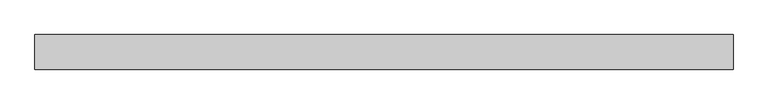
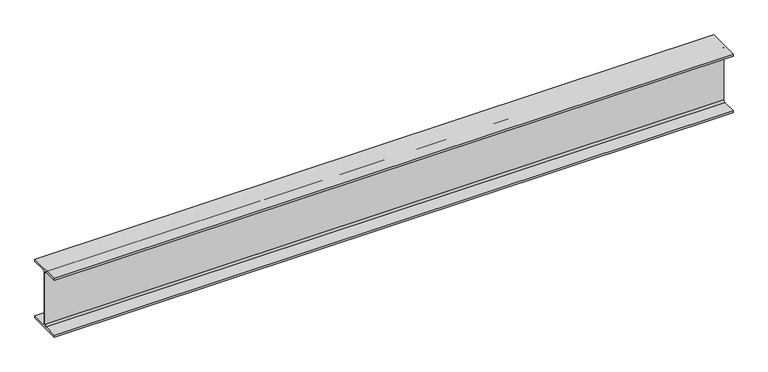
"""IFC4 building model written with IfcOpenShell, lengths in millimetres: beam geometry, Old_Steel Beam_H-KSD3502 : H_SB_ASB_H-200×200x8x12."""

import ifcopenshell
import ifcopenshell.guid

model = None  # the IFC model being written
_history = None  # IfcOwnerHistory: only IFC2X3 demands one
_inside = {}  # id of a spatial element -> (the spatial element, [elements in it])
_under = {}  # id of a project, library or spatial element -> (it, [spatial elements below it])
_declared = {}  # id of a project -> (the project, [libraries it declares])
_typed = {}  # id of a type object -> (the type object, [elements of that type])
_made_of = {}  # id of a material, layer set ... -> (it, [elements and type objects made of it])


def new_model(schema):
    """Start an empty IFC model of exactly this schema.

    Asked for "IFC4X3", IfcOpenShell would pick the latest addendum, in which some entities
    have other attributes; the version numbers below select the first issue.
    IFC2X3 requires an IfcOwnerHistory on every rooted entity: one is made here for all.
    """
    global model, _history
    if schema == "IFC4X3":
        model = ifcopenshell.file(schema_version=(4, 3, 0, 0))
    else:
        model = ifcopenshell.file(schema=schema)
    _inside.clear()
    _under.clear()
    _declared.clear()
    _typed.clear()
    _made_of.clear()
    _history = None
    if model.schema == "IFC2X3":
        org = make("IfcOrganization", Name="unknown")
        user = make(
            "IfcPersonAndOrganization",
            ThePerson=make("IfcPerson", FamilyName="unknown"),
            TheOrganization=org,
        )
        app = make(
            "IfcApplication",
            ApplicationDeveloper=org,
            Version="unknown",
            ApplicationFullName="unknown",
            ApplicationIdentifier="unknown",
        )
        _history = make(
            "IfcOwnerHistory",
            OwningUser=user,
            OwningApplication=app,
            ChangeAction="ADDED",
            CreationDate=0,
        )
    return model


def make(cls, **values):
    """One entity of the class cls with the attributes given. An attribute that is None is left unset."""
    return model.create_entity(
        cls, **{name: value for name, value in values.items() if value is not None}
    )


def rooted(cls, **values):
    """An entity with a GlobalId (a new one), such as an element, a storey or a relation."""
    return make(cls, GlobalId=ifcopenshell.guid.new(), OwnerHistory=_history, **values)


def si_unit(unit_type, name, prefix=None):
    """IfcSIUnit, for example si_unit("LENGTHUNIT", "METRE", prefix="MILLI")."""
    return make("IfcSIUnit", UnitType=unit_type, Prefix=prefix, Name=name)


def assignment(units):
    """IfcUnitAssignment: the units of a project."""
    return None if units is None else make("IfcUnitAssignment", Units=units)


def point(xyz):
    """IfcCartesianPoint."""
    return None if xyz is None else make("IfcCartesianPoint", Coordinates=xyz)


def direction(xyz):
    """IfcDirection."""
    return None if xyz is None else make("IfcDirection", DirectionRatios=xyz)


def frame(location, z_axis=None, x_axis=None):
    """IfcAxis2Placement3D, a coordinate frame: its origin and axes. An axis left out is left unset."""
    return make(
        "IfcAxis2Placement3D",
        Location=point(location),
        Axis=direction(z_axis),
        RefDirection=direction(x_axis),
    )


def frame_2d(location, x_axis=None):
    """IfcAxis2Placement2D, a coordinate frame in the plane: its origin and x axis."""
    return make(
        "IfcAxis2Placement2D", Location=point(location), RefDirection=direction(x_axis)
    )


def origin():
    """The frame at (0, 0, 0) with its axes left unset."""
    return frame((0.0, 0.0, 0.0))


def place(relative_to, where):
    """IfcLocalPlacement: puts the frame where relative to a parent placement (None: the world)."""
    return make(
        "IfcLocalPlacement", PlacementRelTo=relative_to, RelativePlacement=where
    )


def context(
    kind, dimensions, precision=None, world=None, true_north=None, identifier=None
):
    """IfcGeometricRepresentationContext, for example the 3D "Model" context."""
    return make(
        "IfcGeometricRepresentationContext",
        ContextIdentifier=identifier,
        ContextType=kind,
        CoordinateSpaceDimension=dimensions,
        Precision=precision,
        WorldCoordinateSystem=world,
        TrueNorth=true_north,
    )


def project(units=None, contexts=None):
    """IfcProject with its units and contexts."""
    return rooted(
        "IfcProject",
        Name="project",
        RepresentationContexts=contexts,
        UnitsInContext=assignment(units),
    )


def spatial(cls, under=None, at=None, **own):
    """A site, building, storey or space (cls), placed at a placement, below another one or the project."""
    s = rooted(cls, ObjectPlacement=at, **own)
    if under is not None:
        _under.setdefault(under.id(), (under, []))[1].append(s)
    return s


def polyline(points):
    """IfcPolyline through the points."""
    return make("IfcPolyline", Points=[point(p) for p in points])


def circle_curve(where, radius):
    """IfcCircle in the frame where."""
    return make("IfcCircle", Position=where, Radius=radius)


def trimmed(basis, trim1, trim2, sense, master):
    """IfcTrimmedCurve: the piece of a basis curve between two trims."""
    return make(
        "IfcTrimmedCurve",
        BasisCurve=basis,
        Trim1=trim1,
        Trim2=trim2,
        SenseAgreement=sense,
        MasterRepresentation=master,
    )


def segment(curve, same_sense, transition):
    """IfcCompositeCurveSegment."""
    return make(
        "IfcCompositeCurveSegment",
        Transition=transition,
        SameSense=same_sense,
        ParentCurve=curve,
    )


def composite_curve(segments, self_intersect=None):
    """IfcCompositeCurve: segments joined end to end."""
    return make("IfcCompositeCurve", Segments=segments, SelfIntersect=self_intersect)


def outline(outer, holes=None, kind="AREA"):
    """IfcArbitraryClosedProfileDef: a profile drawn as a closed curve; with holes, ...WithVoids."""
    if holes is None:
        return make("IfcArbitraryClosedProfileDef", ProfileType=kind, OuterCurve=outer)
    return make(
        "IfcArbitraryProfileDefWithVoids",
        ProfileType=kind,
        OuterCurve=outer,
        InnerCurves=holes,
    )


def extrude(swept, where, along, depth):
    """IfcExtrudedAreaSolid: the profile swept, set in the frame where, extruded along a direction by depth."""
    return make(
        "IfcExtrudedAreaSolid",
        SweptArea=swept,
        Position=where,
        ExtrudedDirection=direction(along),
        Depth=depth,
    )


def shape(context_of_items, identifier, shape_type, items):
    """IfcShapeRepresentation: the items that make up one representation, for example the "Body"."""
    return make(
        "IfcShapeRepresentation",
        ContextOfItems=context_of_items,
        RepresentationIdentifier=identifier,
        RepresentationType=shape_type,
        Items=items,
    )


def source(mapping_origin, context_of_items, identifier, shape_type, items):
    """IfcRepresentationMap: a shape defined once, which mapped items show again and again."""
    return make(
        "IfcRepresentationMap",
        MappingOrigin=mapping_origin,
        MappedRepresentation=shape(context_of_items, identifier, shape_type, items),
    )


def transform(
    local_origin,
    x_axis=None,
    y_axis=None,
    z_axis=None,
    scale=None,
    scale2=None,
    scale3=None,
    uniform=True,
):
    """IfcCartesianTransformationOperator3D, or its non-uniform kind. x_axis, y_axis, z_axis: its Axis1, 2, 3."""
    if uniform:
        return make(
            "IfcCartesianTransformationOperator3D",
            Axis1=direction(x_axis),
            Axis2=direction(y_axis),
            LocalOrigin=point(local_origin),
            Scale=scale,
            Axis3=direction(z_axis),
        )
    return make(
        "IfcCartesianTransformationOperator3DnonUniform",
        Axis1=direction(x_axis),
        Axis2=direction(y_axis),
        LocalOrigin=point(local_origin),
        Scale=scale,
        Axis3=direction(z_axis),
        Scale2=scale2,
        Scale3=scale3,
    )


def mapped(mapping_source, mapping_target):
    """IfcMappedItem: shows the shape of a source again, moved by a transform."""
    return make(
        "IfcMappedItem", MappingSource=mapping_source, MappingTarget=mapping_target
    )


def made_of(thing, what):
    """Note that an element or type object is made of a material, layer set ...; save() writes the relation."""
    if what is not None:
        _made_of.setdefault(what.id(), (what, []))[1].append(thing)
    return thing


def element(
    cls,
    number,
    at=None,
    inside=None,
    cuts=None,
    type_object=None,
    material=None,
    context=None,
    identifier="Body",
    shape_type=None,
    held_by="IfcProductDefinitionShape",
    body=None,
    shapes=None,
    **own,
):
    """One element of the class cls, such as IfcWall. Its Tag is "e" and its number.

    at: its placement. inside: the storey or other place that contains it. cuts: it is an
    opening in that element (IfcRelVoidsElement). A single representation is given by context,
    identifier, shape_type and body (its items); several are given by shapes. held_by: the class
    of the entity that holds the representations. save() writes the other relations.
    """
    e = rooted(cls, Tag="e%d" % number, ObjectPlacement=at, **own)
    if body is not None:
        shapes = [shape(context, identifier, shape_type, body)]
    if shapes is not None:
        e.Representation = make(held_by, Representations=shapes)
    if inside is not None:
        _inside.setdefault(inside.id(), (inside, []))[1].append(e)
    if cuts is not None:
        rooted(
            "IfcRelVoidsElement", RelatingBuildingElement=cuts, RelatedOpeningElement=e
        )
    if type_object is not None:
        _typed.setdefault(type_object.id(), (type_object, []))[1].append(e)
    return made_of(e, material)


def aggregate(whole, parts):
    """IfcRelAggregates: a whole, such as a stair, and the parts it consists of."""
    return rooted("IfcRelAggregates", RelatingObject=whole, RelatedObjects=parts)


def save(model, path):
    """Write the relations noted so far, then the file.

    IfcRelAggregates (storeys below a building ...), IfcRelContainedInSpatialStructure (elements
    in a storey), IfcRelDefinesByType, IfcRelAssociatesMaterial and IfcRelDeclares: one each for
    every whole, place, type object, material and project.
    """
    for whole, parts in _under.values():
        aggregate(whole, parts)
    for where, things in _inside.values():
        rooted(
            "IfcRelContainedInSpatialStructure",
            RelatedElements=things,
            RelatingStructure=where,
        )
    for kind, things in _typed.values():
        rooted("IfcRelDefinesByType", RelatedObjects=things, RelatingType=kind)
    for what, things in _made_of.values():
        rooted("IfcRelAssociatesMaterial", RelatedObjects=things, RelatingMaterial=what)
    for by, libraries in _declared.values():
        rooted("IfcRelDeclares", RelatingContext=by, RelatedDefinitions=libraries)
    model.write(path)


def beam_fe0ad751(model_context):
    return source(origin(), model_context, "Body", "SweptSolid", [
        extrude(outline(composite_curve([segment(polyline([(82.5, -141.5), (82.5, -151.7), (-82.5, -151.7), (-82.5, -141.5), (-11.9, -141.5)]), True, "CONTINUOUS"), segment(trimmed(circle_curve(frame_2d((-11.9, -132.6)), 8.9), [point((-11.9, -141.5))], [point((-3.0, -132.6))], True, "CARTESIAN"), True, "CONTINUOUS"), segment(polyline([(-3.0, -132.6), (-3.0, 132.6)]), True, "CONTINUOUS"), segment(trimmed(circle_curve(frame_2d((-11.9, 132.6)), 8.9), [point((-3.0, 132.6))], [point((-11.9, 141.5))], True, "CARTESIAN"), True, "CONTINUOUS"), segment(polyline([(-11.9, 141.5), (-82.5, 141.5), (-82.5, 151.7), (82.5, 151.7), (82.5, 141.5), (11.9, 141.5)]), True, "CONTINUOUS"), segment(trimmed(circle_curve(frame_2d((11.9, 132.6)), 8.9), [point((11.9, 141.5))], [point((3.0, 132.6))], True, "CARTESIAN"), True, "CONTINUOUS"), segment(polyline([(3.0, 132.6), (3.0, -132.6)]), True, "CONTINUOUS"), segment(trimmed(circle_curve(frame_2d((11.9, -132.6)), 8.9), [point((3.0, -132.6))], [point((11.9, -141.5))], True, "CARTESIAN"), True, "CONTINUOUS"), segment(polyline([(11.9, -141.5), (82.5, -141.5)]), True, "CONTINUOUS")], self_intersect=False)), frame((-1716.7775834, 0.0, 0.0), z_axis=(1.0, 0.0, 0.0), x_axis=(0.0, 1.0, 0.0)), (0.0, 0.0, 1.0), 3324.8852978),
    ])


if __name__ == "__main__":
    model = new_model("IFC4")
    model_context = context("Model", 3, world=origin())
    ifc_project = project(units=[si_unit("LENGTHUNIT", "METRE", prefix="MILLI")], contexts=[model_context])
    site = spatial("IfcSite", under=ifc_project)
    building = spatial("IfcBuilding", under=site)
    placement = place(None, origin())
    beam_shape = beam_fe0ad751(model_context)
    element("IfcBeam", 1, ObjectType="Old_Steel Beam_H-KSD3502 : H_SB_ASB_H-200×200x8x12", at=placement, inside=building, context=model_context, shape_type="MappedRepresentation", body=[
        mapped(beam_shape, transform((0.0, 0.0, 0.0), x_axis=(1.0, 0.0, 0.0), y_axis=(0.0, 1.0, 0.0), z_axis=(0.0, 0.0, 1.0))),
    ])
    save(model, "model.ifc")

# Revit data of these elements
# Type "Old_Steel Beam_H-KSD3502 : H_SB_ASB_H-200×200x8x12"
#   Width = 20.0 cm
#   Web Thickness = 0.8 cm
#   Web Fillet = 1.3 cm
#   Warping Constant = 141376.0 cm⁶
#   Torsional Moment of Inertia = 26.2485 cm⁴
#   Torsional Modulus = 1.0 cm³
#   Section Area = 63.53 cm²
#   Plastic Modulus weak axis = 244.0 cm³
#   Plastic Modulus strong axis = 525.0 cm³
#   Perimeter = 1.16 m²/m
#   Nominal Weight = 49.90 kgf/m
#   Moment of Inertia weak axis = 1600.00 cm⁴
#   Moment of Inertia strong axis = 4720.00 cm⁴
#   Height = 20.0 cm
#   Flange Thickness = 1.2 cm
#   Elastic Modulus weak axis = 160.0 cm³
#   Elastic Modulus strong axis = 472.0 cm³
#   Centroid Vertical = 10.0 cm
#   Centroid Horizontal = 10.0 cm
#   Length [instance default] = 1.5240 m
#   Structural Material [instance default] = Steel, 45-345
#   Assembly Code = ""
# Element 1 (IfcBeam, "Old_Steel Beam_H-KSD3502 : H_SB_ASB_H-200×200x8x12")
#   Structural Material = none
# Materials
#   "Steel, 45-345": class "Metal", colour RGB 189 187 185, transparency 0, Description = "Steel 345 MPa", Cost = 0
